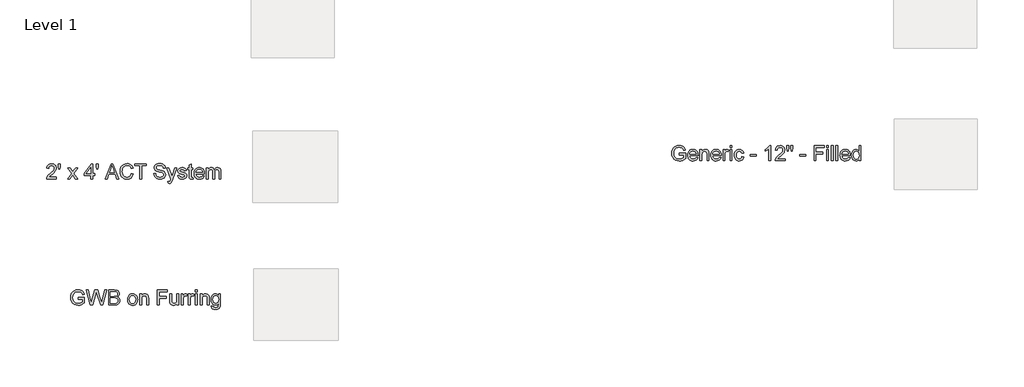
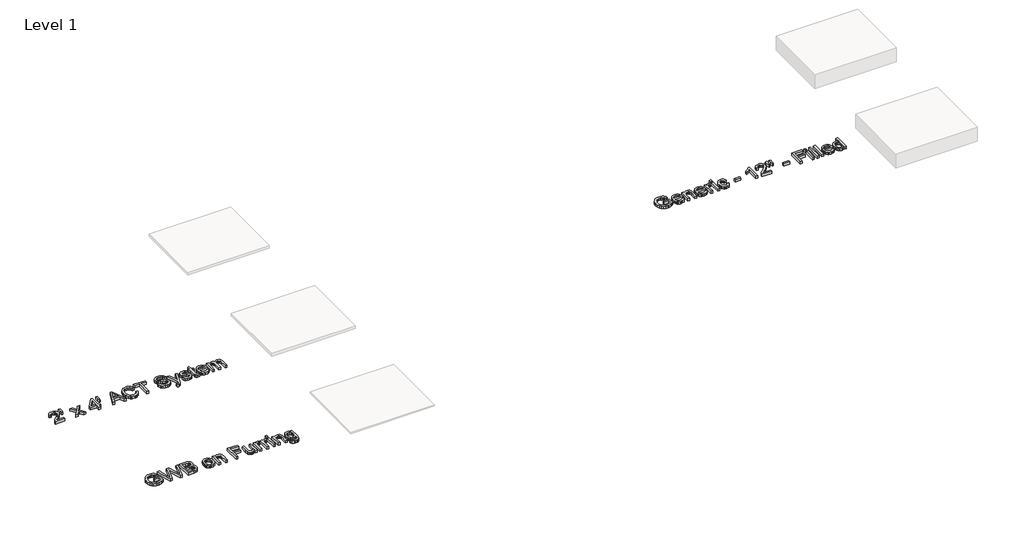
# One storey, part 10 of 42: 3 proxies.
"""IFC4 building model written with IfcOpenShell, lengths in millimetres."""

from ifc_helpers import new_model, si_unit, origin, origin_with_axes, place, context, project, spatial, polyline, outline, extrude, element, save

model = new_model("IFC4")

# Units and contexts
model_context = context("Model", 3, world=origin())
ifc_project = project(units=[si_unit("LENGTHUNIT", "METRE", prefix="MILLI")], contexts=[model_context])

# Site, building, storey
site = spatial("IfcSite", under=ifc_project)
building = spatial("IfcBuilding", under=site)
storey = spatial("IfcBuildingStorey", under=building, Name="Level 1", Elevation=0.0)

# Proxies
placement = place(None, origin())
element("IfcBuildingElementProxy", 1, Name="8\" Arial", ObjectType="8\" Arial", at=placement, inside=storey, context=model_context, shape_type="SweptSolid", body=[
    extrude(outline(polyline([(6877.2165005, -16820.3840044), (6877.2165005, -16858.4548912), (6677.3443451, -16858.4548912), (6681.4339911, -16832.2067993), (6690.8215877, -16811.6935066), (6704.5590805, -16791.7936607), (6724.4310424, -16770.9643499), (6752.2220462, -16747.6626621), (6793.3043995, -16711.1718659), (6817.9538116, -16684.2359699), (6830.2785176, -16662.3749529), (6834.3867529, -16641.1087935), (6830.5108838, -16622.0454662), (6818.8832766, -16606.1980878), (6801.0096645, -16595.5185348), (6778.3957808, -16591.9586839), (6754.6479498, -16595.434883), (6736.1980694, -16605.8634804), (6724.2916226, -16622.4265468), (6720.1740927, -16644.3061532), (6682.1032059, -16639.5472923), (6685.3772464, -16619.8937547), (6691.3327934, -16602.7218887), (6699.969847, -16588.0316942), (6711.2884072, -16575.8231713), (6725.0282237, -16566.2264451), (6740.9290463, -16559.3716407), (6779.21371, -16553.8877971), (6799.6177906, -16555.4121197), (6817.7772132, -16559.9850876), (6833.6919778, -16567.6067006), (6847.3620845, -16578.2769589), (6858.3413899, -16591.2058172), (6866.1837509, -16605.6032302), (6870.8891675, -16621.4691979), (6872.4576397, -16638.8037203), (6870.7660134, -16657.0119398), (6865.6911344, -16674.9041412), (6856.6846185, -16693.1030661), (6843.1980812, -16712.231456), (6821.6995556, -16735.0684113), (6788.6570745, -16764.3930323), (6744.8606833, -16801.0139536), (6727.6841699, -16820.3840044), (6877.2165005, -16820.3840044)])), origin_with_axes(), (0.0, 0.0, 1.0), 50.8),
    extrude(outline(polyline([(6923.8384654, -16663.3415965), (6915.2873873, -16605.5660516), (6915.2873873, -16553.8877971), (6953.3582741, -16553.8877971), (6953.3582741, -16605.5660516), (6944.43541, -16663.3415965), (6923.8384654, -16663.3415965)])), origin_with_axes(), (0.0, 0.0, 1.0), 50.8),
    extrude(outline(polyline([(7100.8829602, -16858.4548912), (7182.2297378, -16746.0268037), (7105.6418211, -16634.7884315), (7151.4458567, -16634.7884315), (7188.4013855, -16688.325616), (7205.652256, -16713.6070642), (7220.5980534, -16692.9357624), (7262.684229, -16634.7884315), (7308.4882646, -16634.7884315), (7228.0337734, -16746.0268037), (7305.5139766, -16858.4548912), (7259.7099409, -16858.4548912), (7213.0879761, -16790.8641957), (7204.536898, -16778.5209004), (7146.6869959, -16858.4548912), (7100.8829602, -16858.4548912)])), origin_with_axes(), (0.0, 0.0, 1.0), 50.8),
    extrude(outline(polyline([(7572.0101839, -16858.4548912), (7572.0101839, -16787.0719785), (7434.0032194, -16787.0719785), (7434.0032194, -16749.0010917), (7581.5279056, -16558.6466579), (7610.0810706, -16558.6466579), (7610.0810706, -16749.0010917), (7648.1519574, -16749.0010917), (7648.1519574, -16787.0719785), (7610.0810706, -16787.0719785), (7610.0810706, -16858.4548912), (7572.0101839, -16858.4548912)]), holes=[polyline([(7572.0101839, -16749.0010917), (7572.0101839, -16631.3680002), (7480.8482558, -16749.0010917), (7572.0101839, -16749.0010917)])]), origin_with_axes(), (0.0, 0.0, 1.0), 50.8),
    extrude(outline(polyline([(7690.0150614, -16663.3415965), (7681.4639833, -16605.5660516), (7681.4639833, -16553.8877971), (7719.5348701, -16553.8877971), (7719.5348701, -16605.5660516), (7710.612006, -16663.3415965), (7690.0150614, -16663.3415965)])), origin_with_axes(), (0.0, 0.0, 1.0), 50.8),
    extrude(outline(polyline([(7860.1443366, -16858.4548912), (7981.7183597, -16553.8877971), (8014.1380992, -16553.8877971), (8135.7121224, -16858.4548912), (8095.4848768, -16858.4548912), (8060.6113497, -16763.2776743), (7935.1707521, -16763.2776743), (7900.3715822, -16858.4548912), (7860.1443366, -16858.4548912)]), holes=[polyline([(7949.1499058, -16725.2067875), (8046.7065531, -16725.2067875), (8019.2687461, -16650.3290864), (7997.9282295, -16591.9586839), (7978.9671433, -16643.7856527), (7949.1499058, -16725.2067875)])]), origin_with_axes(), (0.0, 0.0, 1.0), 50.8),
    extrude(outline(polyline([(8390.5342492, -16750.190807), (8428.6051359, -16760.0059574), (8421.071822, -16783.6817549), (8411.0382473, -16804.3693223), (8398.5044116, -16822.0686597), (8383.4703151, -16836.7797672), (8366.2752125, -16848.3446355), (8347.2583584, -16856.6052558), (8326.4197529, -16861.561628), (8303.759396, -16863.213752), (8259.6005134, -16858.2132303), (8240.929885, -16851.9625781), (8224.5317986, -16843.211665), (8197.6516706, -16818.7295567), (8178.0585482, -16785.2874057), (8166.0963335, -16745.9710358), (8162.1089286, -16703.8662709), (8166.6168339, -16659.4564328), (8180.1405498, -16621.1067065), (8201.9736829, -16590.0346913), (8231.4098397, -16567.4579862), (8266.3205454, -16553.7111988), (8304.5773252, -16549.1289363), (8326.3523667, -16550.6114329), (8346.3195987, -16555.058923), (8364.4790213, -16562.4714065), (8380.8306345, -16572.8488833), (8395.1048934, -16585.9171613), (8407.0322531, -16601.4020484), (8423.8462751, -16639.6216495), (8385.7753883, -16648.693228), (8372.5769852, -16620.9301082), (8354.545364, -16601.8853702), (8331.4574532, -16590.8712098), (8303.0901812, -16587.199823), (8270.3916022, -16591.2708798), (8243.5300634, -16603.48405), (8223.1468958, -16622.5566719), (8209.8834301, -16647.206084), (8202.6057191, -16675.0714449), (8200.1798154, -16703.7919137), (8203.0518623, -16738.9628696), (8211.6680029, -16769.3749647), (8226.35355, -16793.8663677), (8247.4338164, -16811.2752473), (8272.70597, -16821.6759608), (8299.9671787, -16825.1428653), (8331.7455874, -16820.421183), (8358.2260455, -16806.2561363), (8378.2188378, -16782.7964395), (8390.5342492, -16750.190807)])), origin_with_axes(), (0.0, 0.0, 1.0), 50.8),
    extrude(outline(polyline([(8557.0943788, -16858.4548912), (8557.0943788, -16591.9586839), (8457.158301, -16591.9586839), (8457.158301, -16553.8877971), (8695.1013433, -16553.8877971), (8695.1013433, -16591.9586839), (8595.1652655, -16591.9586839), (8595.1652655, -16858.4548912), (8557.0943788, -16858.4548912)])), origin_with_axes(), (0.0, 0.0, 1.0), 50.8),
    extrude(outline(polyline([(8842.6260294, -16753.7599526), (8880.6969162, -16753.7599526), (8885.0654017, -16774.8866922), (8892.9658543, -16791.8680179), (8905.2905603, -16805.3452606), (8922.9318062, -16815.959751), (8944.4953944, -16822.8470867), (8968.5871274, -16825.1428653), (8989.7975189, -16823.4047657), (9008.3682298, -16818.190467), (9023.4162683, -16809.9368177), (9034.0586426, -16799.0806664), (9040.3882994, -16786.6165406), (9042.4981849, -16773.538968), (9040.9180944, -16760.7960027), (9036.1778229, -16749.7818423), (9026.5485654, -16740.3849511), (9010.301517, -16732.4937932), (8954.8682239, -16717.9569604), (8918.4796688, -16708.3369976), (8895.1965703, -16699.1817673), (8876.2447788, -16686.3737395), (8862.8140094, -16670.8516738), (8854.8113157, -16652.9501777), (8852.1437511, -16633.0038586), (8855.4433519, -16610.7059931), (8865.3421543, -16589.9138608), (8881.579908, -16572.2912043), (8903.8963628, -16559.5017658), (8930.6835444, -16551.7221436), (8960.3334782, -16549.1289363), (8992.4557889, -16551.8429741), (9020.5628107, -16559.9850876), (9043.6507215, -16573.387973), (9060.7156991, -16591.8843267), (9071.5160825, -16614.321612), (9075.8102108, -16639.5472923), (9037.7393241, -16639.5472923), (9030.7497472, -16616.8311675), (9016.1757359, -16600.4354047), (8993.4038432, -16590.5087184), (8961.8206222, -16587.199823), (8929.4938292, -16590.4715398), (8907.3167941, -16600.2866903), (8894.4901769, -16614.7305766), (8890.2146379, -16631.8885006), (8893.2446938, -16646.5182799), (8902.3348616, -16658.2853069), (8923.8240926, -16668.8068508), (8964.4974814, -16679.5514663), (9006.4721212, -16689.7569921), (9031.8651052, -16698.6612669), (9053.5681132, -16712.4731169), (9068.7090982, -16729.5195052), (9077.6040783, -16749.6145386), (9080.5690717, -16772.5723244), (9077.1579351, -16796.0413158), (9066.9245254, -16818.1161098), (9050.2871017, -16837.1143746), (9027.6639234, -16851.3537785), (9000.4584826, -16860.2487586), (8970.0742714, -16863.213752), (8932.7748406, -16860.0163924), (8902.0746114, -16850.4243135), (8877.620387, -16834.4003367), (8859.0589708, -16811.9072835), (8847.1432294, -16784.5066551), (8842.6260294, -16753.7599526)])), origin_with_axes(), (0.0, 0.0, 1.0), 50.8),
    extrude(outline(polyline([(9132.916541, -16944.1143864), (9128.1576801, -16907.4562864), (9147.4905523, -16910.8023605), (9165.5593521, -16906.6011786), (9176.638575, -16894.8899195), (9187.0485831, -16866.8572549), (9190.0228711, -16857.636962), (9109.1222368, -16634.7884315), (9149.2751251, -16634.7884315), (9192.1792299, -16758.9649566), (9207.1250273, -16808.6355667), (9222.0708246, -16764.7648183), (9266.1646446, -16634.7884315), (9306.0201042, -16634.7884315), (9228.1681151, -16863.8086096), (9207.9429565, -16913.4792197), (9197.5887163, -16929.3358927), (9185.8588679, -16940.3221691), (9172.2329108, -16946.7354777), (9156.1903448, -16948.8732472), (9132.916541, -16944.1143864)])), origin_with_axes(), (0.0, 0.0, 1.0), 50.8),
    extrude(outline(polyline([(9323.2709748, -16791.8308393), (9361.3418615, -16787.0719785), (9367.3462055, -16803.3562055), (9378.9645181, -16815.3277148), (9396.2711566, -16822.6890776), (9419.3404781, -16825.1428653), (9442.1309601, -16822.8935599), (9458.1549368, -16816.145644), (9467.6354799, -16806.3676721), (9470.795661, -16795.028199), (9467.6168906, -16785.3245843), (9458.0805796, -16777.9260428), (9418.8943349, -16767.0698915), (9361.5649331, -16748.4434127), (9347.0559843, -16739.0837001), (9336.5437351, -16726.6939315), (9330.1583105, -16712.0641523), (9328.0298356, -16695.9844076), (9329.7400512, -16681.233798), (9334.8706981, -16667.6171356), (9342.9570437, -16655.6735102), (9353.5343555, -16645.9420116), (9377.7376243, -16634.6768957), (9410.4919712, -16630.0295706), (9435.2715083, -16631.8977953), (9456.8165072, -16637.5024693), (9474.141735, -16646.2952083), (9486.2619587, -16657.7276279), (9494.2925364, -16672.6455413), (9499.348826, -16691.8947616), (9461.2779393, -16696.6536224), (9456.4726052, -16684.6728185), (9446.9641781, -16675.6477132), (9432.6597116, -16669.9872713), (9413.4662592, -16668.1004574), (9391.6052422, -16669.9036195), (9377.0312309, -16675.3131058), (9368.8333495, -16683.1206119), (9366.1007224, -16692.1178332), (9370.6365116, -16703.1970561), (9384.8387369, -16711.5994198), (9417.6302625, -16719.7043547), (9473.5096988, -16737.62444), (9488.2696031, -16746.1941074), (9499.4603618, -16757.9239558), (9506.5150012, -16772.8511639), (9508.8665477, -16791.0129101), (9506.1060366, -16809.7881033), (9497.8245034, -16827.4479385), (9484.3379661, -16842.6075128), (9465.9624429, -16853.8819233), (9443.7668185, -16860.8807948), (9418.8199777, -16863.213752), (9380.4330728, -16858.7151414), (9352.4189974, -16845.2193094), (9333.7181615, -16822.8749706), (9323.2709748, -16791.8308393)])), origin_with_axes(), (0.0, 0.0, 1.0), 50.8),
    extrude(outline(polyline([(9632.5969297, -16826.7043665), (9637.3557905, -16859.5702492), (9608.8769827, -16863.213752), (9590.6037006, -16861.6336615), (9576.9777436, -16856.89339), (9567.3484861, -16849.587795), (9561.0653026, -16840.3117342), (9557.6076928, -16824.380704), (9556.4551562, -16797.1102006), (9556.4551562, -16672.8593182), (9527.9019911, -16672.8593182), (9527.9019911, -16634.7884315), (9556.4551562, -16634.7884315), (9556.4551562, -16580.4333178), (9594.5260429, -16558.0518003), (9594.5260429, -16634.7884315), (9632.5969297, -16634.7884315), (9632.5969297, -16672.8593182), (9594.5260429, -16672.8593182), (9594.5260429, -16795.9948426), (9596.5336873, -16815.6251436), (9603.0399424, -16822.5775418), (9616.0152739, -16825.1428653), (9632.5969297, -16826.7043665)])), origin_with_axes(), (0.0, 0.0, 1.0), 50.8),
    extrude(outline(polyline([(9827.2640811, -16791.8308393), (9864.5913959, -16796.5897002), (9851.1420372, -16824.7153114), (9829.6806901, -16845.7398099), (9800.6906765, -16858.8452665), (9764.6553181, -16863.213752), (9741.0329649, -16861.3292617), (9719.9852298, -16855.6757908), (9701.5121128, -16846.2533393), (9685.6136138, -16833.0619071), (9672.8288226, -16816.4686331), (9663.6968289, -16796.8406557), (9658.2176326, -16774.1779752), (9656.3912339, -16748.4805913), (9658.2362219, -16721.9118341), (9663.7711861, -16698.4939632), (9672.9961263, -16678.2269786), (9685.9110426, -16661.1108805), (9701.7677156, -16647.5128074), (9719.8179261, -16637.7998981), (9740.061674, -16631.9721525), (9762.4989593, -16630.0295706), (9784.2135856, -16631.9675052), (9803.8508575, -16637.7813088), (9821.4107752, -16647.4709815), (9836.8933386, -16661.0365233), (9849.5317391, -16678.1154428), (9858.559168, -16698.3452488), (9863.9756253, -16721.7259411), (9865.7811111, -16748.2575197), (9865.5580395, -16758.5188134), (9694.4621207, -16758.5188134), (9701.0520276, -16787.0162106), (9716.3603163, -16807.9663519), (9738.4536995, -16820.8487369), (9765.3988901, -16825.1428653), (9785.6612273, -16823.1538101), (9802.7262049, -16817.1866448), (9816.5938228, -16806.8695832), (9827.2640811, -16791.8308393)]), holes=[polyline([(9694.4621207, -16720.4479267), (9827.7102243, -16720.4479267), (9822.5609882, -16700.3343039), (9812.4669982, -16685.9461855), (9790.2713738, -16672.5618894), (9762.3502449, -16668.1004574), (9736.687716, -16671.6603084), (9715.4680299, -16682.3398613), (9700.7174202, -16698.9865796), (9694.4621207, -16720.4479267)])]), origin_with_axes(), (0.0, 0.0, 1.0), 50.8),
    extrude(outline(polyline([(9903.8519978, -16858.4548912), (9903.8519978, -16634.7884315), (9941.9228846, -16634.7884315), (9941.9228846, -16671.5952458), (9953.3738935, -16654.6882773), (9968.0966192, -16641.4434009), (9985.5891507, -16632.8830282), (10005.3495768, -16630.0295706), (10026.5227897, -16632.9387961), (10043.4948208, -16641.6664725), (10056.1727235, -16655.6363316), (10064.4635513, -16674.272105), (10078.3404639, -16654.9159962), (10094.169253, -16641.0902042), (10111.9499186, -16632.794729), (10131.6824608, -16630.0295706), (10160.3006884, -16634.6304224), (10181.4646067, -16648.4329778), (10194.5421793, -16671.8090228), (10198.9013702, -16705.1303433), (10198.9013702, -16858.4548912), (10160.8304835, -16858.4548912), (10160.8304835, -16721.4889275), (10157.2985164, -16689.7012242), (10152.3351733, -16680.9363691), (10144.5090779, -16674.0490334), (10134.4429719, -16669.5876014), (10122.7595967, -16668.1004574), (10102.1347682, -16671.9112639), (10085.3207461, -16683.3436835), (10074.1392821, -16703.1784668), (10070.4121274, -16732.1963644), (10070.4121274, -16858.4548912), (10032.3412406, -16858.4548912), (10032.3412406, -16717.250567), (10030.1384086, -16695.7241574), (10023.5299124, -16680.3693955), (10011.9023051, -16671.1676919), (9994.6421399, -16668.1004574), (9979.9751821, -16670.1452804), (9966.4607608, -16676.2797495), (9955.3071807, -16686.3551502), (9947.7227463, -16700.2227681), (9943.37285, -16719.4626938), (9941.9228846, -16745.6550177), (9941.9228846, -16858.4548912), (9903.8519978, -16858.4548912)])), origin_with_axes(), (0.0, 0.0, 1.0), 50.8),
])
element("IfcBuildingElementProxy", 2, Name="8\" Arial", ObjectType="8\" Arial", at=placement, inside=storey, context=model_context, shape_type="SweptSolid", body=[
    extrude(outline(polyline([(7319.6329177, -19290.0141217), (7319.6329177, -19251.943235), (7443.3632997, -19251.943235), (7443.3632997, -19365.7841092), (7413.2951067, -19386.6970719), (7382.2788593, -19401.6986372), (7350.3889149, -19410.7330371), (7317.6996305, -19413.7445037), (7274.9907134, -19408.9577589), (7236.3900315, -19394.5975245), (7204.3234887, -19371.1657116), (7181.2169886, -19339.1642314), (7167.2471295, -19300.7773265), (7162.5905098, -19258.1892398), (7167.2285402, -19215.2944297), (7181.1426314, -19175.3924968), (7203.7565151, -19141.9224619), (7218.1097785, -19128.8890388), (7234.4939229, -19118.3233453), (7271.9327735, -19104.3256023), (7314.6509853, -19099.6596879), (7346.0111347, -19102.3644311), (7374.211103, -19110.4786606), (7397.958934, -19123.4168135), (7415.9626712, -19140.5933269), (7429.2819048, -19162.8354246), (7438.9762248, -19190.9703304), (7403.8796261, -19200.8598381), (7396.0442361, -19180.7926885), (7386.5172198, -19165.6517035), (7373.9136742, -19154.2378732), (7356.8486967, -19145.3521878), (7336.5027076, -19139.635978), (7314.0561277, -19137.7305747), (7287.7801519, -19139.7846924), (7265.3149826, -19145.9470454), (7246.7442717, -19155.4461778), (7232.1516711, -19167.5106336), (7212.5585487, -19196.8445492), (7203.6356846, -19225.5836073), (7200.6613966, -19256.6277386), (7204.2398369, -19293.034883), (7214.9751577, -19322.9915402), (7232.5420464, -19346.2839333), (7256.6151901, -19362.6982854), (7284.7872745, -19372.429784), (7314.6509853, -19375.6736169), (7341.0199076, -19373.229124), (7366.7382044, -19365.895645), (7389.0732485, -19355.7923604), (7405.2924129, -19345.0384502), (7405.2924129, -19290.0141217), (7319.6329177, -19290.0141217)])), origin_with_axes(), (0.0, 0.0, 1.0), 50.8),
    extrude(outline(polyline([(7559.7323188, -19408.9856428), (7476.6753256, -19104.4185488), (7515.9359276, -19104.4185488), (7564.1193936, -19304.5881331), (7578.9908338, -19366.3789668), (7594.9032747, -19311.7264243), (7655.2813217, -19104.4185488), (7711.8671514, -19104.4185488), (7755.7378998, -19254.6944514), (7774.5316823, -19310.4623519), (7788.3807109, -19366.3789668), (7802.8060079, -19306.3727059), (7851.4356171, -19104.4185488), (7890.6962191, -19104.4185488), (7807.5648687, -19408.9856428), (7766.8914799, -19408.9856428), (7693.8727088, -19174.0168886), (7683.6857724, -19141.2253631), (7672.2347634, -19180.7090367), (7605.6850688, -19408.9856428), (7559.7323188, -19408.9856428)])), origin_with_axes(), (0.0, 0.0, 1.0), 50.8),
    extrude(outline(polyline([(7928.7671059, -19408.9856428), (7928.7671059, -19104.4185488), (8044.9874106, -19104.4185488), (8076.9517122, -19106.6585594), (8101.9078477, -19113.3785915), (8121.0362376, -19124.7459485), (8135.5173024, -19140.9279343), (8144.6353541, -19159.9633777), (8147.6747047, -19179.8911075), (8145.1186759, -19198.2294521), (8137.4505896, -19215.471028), (8124.6146779, -19230.5562451), (8106.5551727, -19242.4255133), (8128.1280556, -19253.6906292), (8144.0683805, -19270.8299639), (8153.9114149, -19292.7095702), (8157.1924264, -19318.1955008), (8154.9524157, -19339.4337762), (8148.2323837, -19359.1291398), (8138.2034563, -19375.8780992), (8126.0367593, -19388.2771624), (8111.1374352, -19397.2557944), (8092.9106264, -19403.7434602), (8044.0951241, -19408.9856428), (7928.7671059, -19408.9856428)]), holes=[polyline([(7966.8379926, -19228.1489307), (8036.3619753, -19228.1489307), (8076.9610069, -19224.8772139), (8091.1725268, -19219.2353613), (8101.3873473, -19210.7865244), (8107.5497003, -19199.6608282), (8109.603818, -19185.9883979), (8107.68912, -19172.7156376), (8101.9450263, -19161.1530929), (8092.6317869, -19152.1279877), (8080.0096521, -19146.4675458), (8031.082614, -19142.4894355), (7966.8379926, -19142.4894355), (7966.8379926, -19228.1489307)]), polyline([(7966.8379926, -19370.9147561), (8044.9130534, -19370.9147561), (8073.1687896, -19369.4276121), (8097.0746296, -19361.1367842), (8112.9127134, -19344.220521), (8117.5693331, -19332.267601), (8119.1215397, -19318.5672868), (8117.2997882, -19302.6548458), (8111.834534, -19288.9731209), (8102.2889283, -19278.2749787), (8088.2261228, -19271.3132857), (8068.3076876, -19267.4931846), (8041.1951933, -19266.2198175), (7966.8379926, -19266.2198175), (7966.8379926, -19370.9147561)])]), origin_with_axes(), (0.0, 0.0, 1.0), 50.8),
    extrude(outline(polyline([(8314.2348343, -19297.152413), (8316.2935993, -19268.185636), (8322.4698943, -19243.2248532), (8332.7637192, -19222.2700646), (8347.1750742, -19205.3212701), (8361.684023, -19194.4883554), (8377.6987051, -19186.7505592), (8395.2191205, -19182.1078815), (8414.2452692, -19180.5603223), (8435.2488548, -19182.4448126), (8454.2401486, -19188.0982835), (8471.2191506, -19197.520735), (8486.1858609, -19210.7121672), (8498.4013548, -19227.2264367), (8507.1267076, -19246.6174005), (8512.3619192, -19268.8850584), (8514.1069898, -19294.0294106), (8511.0211659, -19332.4906726), (8501.7636945, -19361.7688204), (8486.6041202, -19383.6948999), (8465.8119879, -19400.0999574), (8441.1161026, -19410.3333671), (8414.2452692, -19413.7445037), (8392.9349602, -19411.8669844), (8373.7670681, -19406.2344264), (8356.7415928, -19396.8468298), (8341.8585343, -19383.7041946), (8329.7731656, -19367.0295923), (8321.1407593, -19347.0460947), (8315.9613155, -19323.7537015), (8314.2348343, -19297.152413)]), holes=[polyline([(8352.305721, -19297.0780558), (8356.7113852, -19331.5333237), (8369.9283776, -19356.0804945), (8389.8189288, -19370.7753363), (8414.2452692, -19375.6736169), (8438.5600739, -19370.7474524), (8458.4134464, -19355.9689587), (8471.6304389, -19331.0964751), (8476.036103, -19295.8883406), (8471.6025549, -19262.4368949), (8458.3019106, -19238.2243314), (8438.4206541, -19223.5294896), (8414.2452692, -19218.631209), (8389.8189288, -19223.5109003), (8369.9283776, -19238.1499742), (8356.7113852, -19262.6413772), (8352.305721, -19297.0780558)])]), origin_with_axes(), (0.0, 0.0, 1.0), 50.8),
    extrude(outline(polyline([(8556.9367374, -19408.9856428), (8556.9367374, -19185.3191831), (8595.0076241, -19185.3191831), (8595.0076241, -19216.5492074), (8608.2339112, -19200.8040702), (8624.1184682, -19189.5575436), (8642.6612951, -19182.8096276), (8663.862392, -19180.5603223), (8682.6282905, -19182.3727791), (8699.8140985, -19187.8101494), (8714.146449, -19196.1939237), (8724.3519748, -19206.8455927), (8735.7658051, -19234.8410788), (8737.7734495, -19271.6478931), (8737.7734495, -19408.9856428), (8699.7025627, -19408.9856428), (8699.7025627, -19276.77854), (8695.3154879, -19243.0947281), (8689.2460814, -19233.0658006), (8679.8120115, -19225.2861785), (8667.7196718, -19220.2949514), (8653.6754555, -19218.631209), (8631.3775899, -19222.3676584), (8612.3700305, -19233.5770064), (8604.7739777, -19242.7275894), (8599.3482257, -19255.2335411), (8595.0076241, -19290.3115505), (8595.0076241, -19408.9856428), (8556.9367374, -19408.9856428)])), origin_with_axes(), (0.0, 0.0, 1.0), 50.8),
    extrude(outline(polyline([(8913.8513007, -19408.9856428), (8913.8513007, -19104.4185488), (9118.4823171, -19104.4185488), (9118.4823171, -19142.4894355), (8951.9221875, -19142.4894355), (8951.9221875, -19232.9077916), (9094.6880128, -19232.9077916), (9094.6880128, -19270.9786783), (8951.9221875, -19270.9786783), (8951.9221875, -19408.9856428), (8913.8513007, -19408.9856428)])), origin_with_axes(), (0.0, 0.0, 1.0), 50.8),
    extrude(outline(polyline([(9308.8367509, -19408.9856428), (9308.8367509, -19370.5429701), (9295.0620794, -19389.443641), (9279.0195134, -19402.9441203), (9260.7090527, -19411.0444078), (9240.1306974, -19413.7445037), (9221.5878705, -19411.8483951), (9204.3277053, -19406.1600692), (9189.8466404, -19397.6089911), (9179.6411146, -19387.1246258), (9172.7723682, -19374.3909552), (9168.3016415, -19359.0919612), (9166.0709255, -19323.6979336), (9166.0709255, -19185.3191831), (9204.1418123, -19185.3191831), (9204.1418123, -19305.7778483), (9206.4468855, -19344.592307), (9211.9957916, -19357.5397546), (9221.5042186, -19367.382789), (9234.3401304, -19373.60091), (9249.8714907, -19375.6736169), (9266.2951374, -19373.5544367), (9281.659194, -19367.196896), (9294.3278021, -19357.1865579), (9302.6651032, -19344.1089852), (9307.2938389, -19326.1981945), (9308.8367509, -19301.6882022), (9308.8367509, -19185.3191831), (9346.9076376, -19185.3191831), (9346.9076376, -19408.9856428), (9308.8367509, -19408.9856428)])), origin_with_axes(), (0.0, 0.0, 1.0), 50.8),
    extrude(outline(polyline([(9399.2551069, -19408.9856428), (9399.2551069, -19185.3191831), (9432.5671328, -19185.3191831), (9432.5671328, -19218.4081374), (9444.8732495, -19199.2239797), (9456.2127226, -19187.9216852), (9467.5893744, -19182.400663), (9480.0070269, -19180.5603223), (9498.968113, -19183.4974317), (9518.226628, -19192.30876), (9505.5115467, -19226.4387151), (9492.1272506, -19220.5830856), (9478.7429545, -19218.631209), (9467.3755974, -19220.5087284), (9457.2165449, -19226.1412863), (9449.0093688, -19235.101329), (9443.4976413, -19246.9613025), (9438.8689056, -19268.2274619), (9437.3259937, -19291.4269085), (9437.3259937, -19408.9856428), (9399.2551069, -19408.9856428)])), origin_with_axes(), (0.0, 0.0, 1.0), 50.8),
    extrude(outline(polyline([(9542.0209323, -19408.9856428), (9542.0209323, -19185.3191831), (9575.3329582, -19185.3191831), (9575.3329582, -19218.4081374), (9587.6390749, -19199.2239797), (9598.978548, -19187.9216852), (9610.3551997, -19182.400663), (9622.7728522, -19180.5603223), (9641.7339384, -19183.4974317), (9660.9924534, -19192.30876), (9648.2773721, -19226.4387151), (9634.8930759, -19220.5830856), (9621.5087798, -19218.631209), (9610.1414227, -19220.5087284), (9599.9823702, -19226.1412863), (9591.7751942, -19235.101329), (9586.2634667, -19246.9613025), (9581.6347309, -19268.2274619), (9580.091819, -19291.4269085), (9580.091819, -19408.9856428), (9542.0209323, -19408.9856428)])), origin_with_axes(), (0.0, 0.0, 1.0), 50.8),
    extrude(outline(polyline([(9684.7867576, -19142.4894355), (9684.7867576, -19104.4185488), (9722.8576444, -19104.4185488), (9722.8576444, -19142.4894355), (9684.7867576, -19142.4894355)])), origin_with_axes(), (0.0, 0.0, 1.0), 50.8),
    extrude(outline(polyline([(9684.7867576, -19408.9856428), (9684.7867576, -19185.3191831), (9722.8576444, -19185.3191831), (9722.8576444, -19408.9856428), (9684.7867576, -19408.9856428)])), origin_with_axes(), (0.0, 0.0, 1.0), 50.8),
    extrude(outline(polyline([(9779.9639745, -19408.9856428), (9779.9639745, -19185.3191831), (9818.0348613, -19185.3191831), (9818.0348613, -19216.5492074), (9831.2611483, -19200.8040702), (9847.1457053, -19189.5575436), (9865.6885323, -19182.8096276), (9886.8896291, -19180.5603223), (9905.6555276, -19182.3727791), (9922.8413356, -19187.8101494), (9937.1736861, -19196.1939237), (9947.3792119, -19206.8455927), (9958.7930422, -19234.8410788), (9960.8006866, -19271.6478931), (9960.8006866, -19408.9856428), (9922.7297998, -19408.9856428), (9922.7297998, -19276.77854), (9918.342725, -19243.0947281), (9912.2733185, -19233.0658006), (9902.8392487, -19225.2861785), (9890.7469089, -19220.2949514), (9876.7026926, -19218.631209), (9854.404827, -19222.3676584), (9835.3972676, -19233.5770064), (9827.8012148, -19242.7275894), (9822.3754628, -19255.2335411), (9818.0348613, -19290.3115505), (9818.0348613, -19408.9856428), (9779.9639745, -19408.9856428)])), origin_with_axes(), (0.0, 0.0, 1.0), 50.8),
    extrude(outline(polyline([(10003.6304342, -19428.0210862), (10041.701321, -19432.7799471), (10045.9025028, -19444.6770992), (10054.0446163, -19452.8563913), (10070.0500037, -19459.2139319), (10091.000145, -19461.3331121), (10113.3444838, -19458.9350924), (10129.9633182, -19451.7410332), (10141.4886843, -19440.2156671), (10148.5526184, -19424.8237266), (10151.1551204, -19380.4324778), (10138.4865123, -19392.9244875), (10124.3493495, -19401.8473516), (10108.743632, -19407.20107), (10091.6693598, -19408.9856428), (10070.7958994, -19406.9082885), (10052.4180525, -19400.6762257), (10036.5358192, -19390.2894542), (10023.1491994, -19375.7479741), (10012.527738, -19358.3019159), (10004.9409799, -19339.20141), (10000.388925, -19318.4464563), (9998.8715734, -19296.037055), (10001.5949058, -19265.2996471), (10009.7649033, -19237.0346162), (10023.0934315, -19213.0823029), (10041.2923564, -19195.283048), (10063.7389363, -19184.2410037), (10089.8104298, -19180.5603223), (10107.6143321, -19182.6423239), (10123.7730812, -19188.8883288), (10138.2866773, -19199.2983369), (10151.1551204, -19213.8723482), (10151.1551204, -19185.3191831), (10189.2260071, -19185.3191831), (10189.2260071, -19378.4248333), (10186.6235051, -19423.0112698), (10178.815999, -19452.3730694), (10165.3666404, -19471.8453614), (10145.8385805, -19486.7632748), (10120.6593735, -19496.2438179), (10090.256573, -19499.4039989), (10054.8346615, -19494.9518615), (10026.9414166, -19481.5954493), (10016.4361384, -19471.5688455), (10009.0492152, -19459.2975838), (10004.7806471, -19444.781664), (10003.6304342, -19428.0210862)]), holes=[polyline([(10036.9424601, -19293.4345529), (10041.0042222, -19328.3545533), (10053.1895085, -19352.3626345), (10071.5092638, -19366.2767257), (10093.9744331, -19370.9147561), (10116.2722986, -19366.3046096), (10134.6850004, -19352.4741703), (10147.0375904, -19328.7728126), (10151.1551204, -19294.549911), (10146.9167599, -19261.5446085), (10134.2016786, -19237.7781882), (10115.519432, -19223.4179538), (10093.3795754, -19218.631209), (10071.6393889, -19223.3435966), (10053.4125801, -19237.4807594), (10041.0599901, -19260.893983), (10036.9424601, -19293.4345529)])]), origin_with_axes(), (0.0, 0.0, 1.0), 50.8),
])
element("IfcBuildingElementProxy", 3, Name="8\" Arial", ObjectType="8\" Arial", at=placement, inside=storey, context=model_context, shape_type="SweptSolid", body=[
    extrude(outline(polyline([(19456.3608606, -16371.1352359), (19456.3608606, -16333.0643492), (19580.0912426, -16333.0643492), (19580.0912426, -16446.9052234), (19550.0230495, -16467.8181861), (19519.0068022, -16482.8197514), (19487.1168577, -16491.8541513), (19454.4275734, -16494.8656179), (19411.7186562, -16490.0788731), (19373.1179744, -16475.7186387), (19341.0514316, -16452.2868258), (19317.9449315, -16420.2853456), (19303.9750724, -16381.8984407), (19299.3184527, -16339.310354), (19303.9564831, -16296.4155439), (19317.8705743, -16256.5136111), (19340.484458, -16223.0435761), (19354.8377214, -16210.010153), (19371.2218658, -16199.4444595), (19408.6607164, -16185.4467165), (19451.3789282, -16180.7808021), (19482.7390776, -16183.4855453), (19510.9390459, -16191.5997748), (19534.6868769, -16204.5379278), (19552.6906141, -16221.7144411), (19566.0098477, -16243.9565388), (19575.7041677, -16272.0914446), (19540.607569, -16281.9809523), (19532.772179, -16261.9138028), (19523.2451626, -16246.7728178), (19510.6416171, -16235.3589875), (19493.5766396, -16226.473302), (19473.2306505, -16220.7570922), (19450.7840706, -16218.8516889), (19424.5080948, -16220.9058066), (19402.0429255, -16227.0681596), (19383.4722146, -16236.567292), (19368.879614, -16248.6317478), (19349.2864916, -16277.9656635), (19340.3636275, -16306.7047215), (19337.3893395, -16337.7488528), (19340.9677798, -16374.1559972), (19351.7031006, -16404.1126544), (19369.2699893, -16427.4050476), (19393.343133, -16443.8193996), (19421.5152174, -16453.5508983), (19451.3789282, -16456.7947311), (19477.7478505, -16454.3502382), (19503.4661473, -16447.0167592), (19525.8011914, -16436.9134746), (19542.0203558, -16426.1595645), (19542.0203558, -16371.1352359), (19456.3608606, -16371.1352359)])), origin_with_axes(), (0.0, 0.0, 1.0), 50.8),
    extrude(outline(polyline([(19793.7938374, -16423.4827052), (19831.1211521, -16428.2415661), (19817.6717935, -16456.3671772), (19796.2104464, -16477.3916757), (19767.2204328, -16490.4971324), (19731.1850744, -16494.8656179), (19707.5627212, -16492.9811276), (19686.5149861, -16487.3276567), (19668.041869, -16477.9052052), (19652.1433701, -16464.713773), (19639.3585789, -16448.1204989), (19630.2265851, -16428.4925216), (19624.7473889, -16405.829841), (19622.9209902, -16380.1324572), (19624.7659782, -16353.5636999), (19630.3009423, -16330.145829), (19639.5258826, -16309.8788445), (19652.4407989, -16292.7627464), (19668.2974719, -16279.1646733), (19686.3476824, -16269.451764), (19706.5914303, -16263.6240184), (19729.0287156, -16261.6814365), (19750.7433418, -16263.619371), (19770.3806138, -16269.4331747), (19787.9405315, -16279.1228474), (19803.4230949, -16292.6883892), (19816.0614953, -16309.7673087), (19825.0889242, -16329.9971146), (19830.5053816, -16353.3778069), (19832.3108673, -16379.9093856), (19832.0877957, -16390.1706793), (19660.9918769, -16390.1706793), (19667.5817838, -16418.6680765), (19682.8900725, -16439.6182178), (19704.9834558, -16452.5006028), (19731.9286464, -16456.7947311), (19752.1909836, -16454.805676), (19769.2559612, -16448.8385107), (19783.1235791, -16438.5214491), (19793.7938374, -16423.4827052)]), holes=[polyline([(19660.9918769, -16352.0997926), (19794.2399806, -16352.0997926), (19789.0907444, -16331.9861698), (19778.9967544, -16317.5980514), (19756.80113, -16304.2137553), (19728.8800012, -16299.7523233), (19703.2174723, -16303.3121742), (19681.9977861, -16313.9917272), (19667.2471764, -16330.6384455), (19660.9918769, -16352.0997926)])]), origin_with_axes(), (0.0, 0.0, 1.0), 50.8),
    extrude(outline(polyline([(19870.3817541, -16490.1067571), (19870.3817541, -16266.4402973), (19908.4526409, -16266.4402973), (19908.4526409, -16297.6703216), (19921.6789279, -16281.9251844), (19937.5634849, -16270.6786578), (19956.1063119, -16263.9307418), (19977.3074087, -16261.6814365), (19996.0733072, -16263.4938933), (20013.2591153, -16268.9312636), (20027.5914657, -16277.315038), (20037.7969915, -16287.966707), (20049.2108218, -16315.962193), (20051.2184662, -16352.7690074), (20051.2184662, -16490.1067571), (20013.1475795, -16490.1067571), (20013.1475795, -16357.8996542), (20008.7605046, -16324.2158423), (20002.6910981, -16314.1869148), (19993.2570283, -16306.4072927), (19981.1646885, -16301.4160656), (19967.1204722, -16299.7523233), (19944.8226067, -16303.4887726), (19925.8150472, -16314.6981206), (19918.2189944, -16323.8487036), (19912.7932425, -16336.3546553), (19908.4526409, -16371.4326647), (19908.4526409, -16490.1067571), (19870.3817541, -16490.1067571)])), origin_with_axes(), (0.0, 0.0, 1.0), 50.8),
    extrude(outline(polyline([(20260.1622002, -16423.4827052), (20297.4895149, -16428.2415661), (20284.0401563, -16456.3671772), (20262.5788092, -16477.3916757), (20233.5887956, -16490.4971324), (20197.5534372, -16494.8656179), (20173.931084, -16492.9811276), (20152.8833489, -16487.3276567), (20134.4102318, -16477.9052052), (20118.5117328, -16464.713773), (20105.7269416, -16448.1204989), (20096.5949479, -16428.4925216), (20091.1157517, -16405.829841), (20089.289353, -16380.1324572), (20091.134341, -16353.5636999), (20096.6693051, -16330.145829), (20105.8942454, -16309.8788445), (20118.8091616, -16292.7627464), (20134.6658347, -16279.1646733), (20152.7160452, -16269.451764), (20172.9597931, -16263.6240184), (20195.3970784, -16261.6814365), (20217.1117046, -16263.619371), (20236.7489766, -16269.4331747), (20254.3088943, -16279.1228474), (20269.7914577, -16292.6883892), (20282.4298581, -16309.7673087), (20291.457287, -16329.9971146), (20296.8737444, -16353.3778069), (20298.6792301, -16379.9093856), (20298.4561585, -16390.1706793), (20127.3602397, -16390.1706793), (20133.9501466, -16418.6680765), (20149.2584353, -16439.6182178), (20171.3518186, -16452.5006028), (20198.2970092, -16456.7947311), (20218.5593464, -16454.805676), (20235.6243239, -16448.8385107), (20249.4919419, -16438.5214491), (20260.1622002, -16423.4827052)]), holes=[polyline([(20127.3602397, -16352.0997926), (20260.6083434, -16352.0997926), (20255.4591072, -16331.9861698), (20245.3651172, -16317.5980514), (20223.1694928, -16304.2137553), (20195.248364, -16299.7523233), (20169.5858351, -16303.3121742), (20148.3661489, -16313.9917272), (20133.6155392, -16330.6384455), (20127.3602397, -16352.0997926)])]), origin_with_axes(), (0.0, 0.0, 1.0), 50.8),
    extrude(outline(polyline([(20336.7501169, -16490.1067571), (20336.7501169, -16266.4402973), (20370.0621428, -16266.4402973), (20370.0621428, -16299.5292517), (20382.3682595, -16280.3450939), (20393.7077326, -16269.0427994), (20405.0843843, -16263.5217772), (20417.5020369, -16261.6814365), (20436.463123, -16264.6185459), (20455.721638, -16273.4298742), (20443.0065567, -16307.5598293), (20429.6222606, -16301.7041998), (20416.2379644, -16299.7523233), (20404.8706074, -16301.6298426), (20394.7115548, -16307.2624005), (20386.5043788, -16316.2224432), (20380.9926513, -16328.0824167), (20376.3639156, -16349.3485761), (20374.8210037, -16372.5480227), (20374.8210037, -16490.1067571), (20336.7501169, -16490.1067571)])), origin_with_axes(), (0.0, 0.0, 1.0), 50.8),
    extrude(outline(polyline([(20479.5159422, -16490.1067571), (20479.5159422, -16266.4402973), (20517.586829, -16266.4402973), (20517.586829, -16490.1067571), (20479.5159422, -16490.1067571)])), origin_with_axes(), (0.0, 0.0, 1.0), 50.8),
    extrude(outline(polyline([(20479.5159422, -16223.6105497), (20479.5159422, -16185.539663), (20517.586829, -16185.539663), (20517.586829, -16223.6105497), (20479.5159422, -16223.6105497)])), origin_with_axes(), (0.0, 0.0, 1.0), 50.8),
    extrude(outline(polyline([(20717.4589845, -16409.2061227), (20755.5298712, -16413.9649835), (20744.9153808, -16447.8253938), (20724.9690618, -16473.4135655), (20697.5684333, -16489.5026048), (20664.5910148, -16494.8656179), (20643.2388799, -16492.9950696), (20624.0942244, -16487.3834246), (20607.1570482, -16478.0306829), (20592.4273515, -16464.9368446), (20580.5046391, -16448.3482179), (20571.988416, -16428.5111109), (20566.8786821, -16405.4255238), (20565.1754375, -16379.0914564), (20568.0846629, -16345.2124568), (20576.8123394, -16315.8506572), (20591.4978865, -16292.1400048), (20612.2807241, -16275.214447), (20637.1439131, -16265.0646891), (20664.0705144, -16261.6814365), (20696.2392983, -16266.3287615), (20721.9575951, -16280.2707367), (20740.4074756, -16302.7637899), (20750.7710104, -16333.0643492), (20712.7001236, -16337.82321), (20705.7941986, -16321.2136703), (20695.0402885, -16309.3072236), (20681.0332508, -16302.1410483), (20664.3679432, -16299.7523233), (20639.7650044, -16304.4554162), (20620.2369446, -16318.564695), (20607.4939793, -16342.8423211), (20603.2463242, -16378.0504556), (20607.4010328, -16413.7326173), (20619.8651586, -16438.0938952), (20639.0400217, -16452.1195221), (20663.3269424, -16456.7947311), (20683.0408952, -16453.876211), (20699.2042917, -16445.1206506), (20710.9620241, -16430.3049784), (20717.4589845, -16409.2061227)])), origin_with_axes(), (0.0, 0.0, 1.0), 50.8),
    extrude(outline(polyline([(20888.7779749, -16399.688401), (20888.7779749, -16361.6175142), (21007.749496, -16361.6175142), (21007.749496, -16399.688401), (20888.7779749, -16399.688401)])), origin_with_axes(), (0.0, 0.0, 1.0), 50.8),
    extrude(outline(polyline([(21302.7988684, -16490.1067571), (21264.7279816, -16490.1067571), (21264.7279816, -16252.7585724), (21228.6647393, -16278.4489853), (21188.5862081, -16297.6703216), (21188.5862081, -16261.6814365), (21218.4870975, -16245.4157989), (21244.3912872, -16226.0643374), (21264.8116335, -16205.4859821), (21278.2609922, -16185.539663), (21302.7988684, -16185.539663), (21302.7988684, -16490.1067571)])), origin_with_axes(), (0.0, 0.0, 1.0), 50.8),
    extrude(outline(polyline([(21588.3305191, -16452.0358703), (21588.3305191, -16490.1067571), (21388.4583636, -16490.1067571), (21392.5480096, -16463.8586652), (21401.9356062, -16443.3453725), (21415.6730991, -16423.4455266), (21435.5450609, -16402.6162158), (21463.3360647, -16379.314528), (21504.4184181, -16342.8237318), (21529.0678301, -16315.8878358), (21541.3925361, -16294.0268188), (21545.5007715, -16272.7606594), (21541.6249024, -16253.6973321), (21529.9972951, -16237.8499537), (21512.123683, -16227.1704007), (21489.5097994, -16223.6105497), (21465.7619684, -16227.0867489), (21447.312088, -16237.5153463), (21435.4056412, -16254.0784127), (21431.2881112, -16275.958019), (21393.2172244, -16271.1991582), (21396.4912649, -16251.5456206), (21402.446812, -16234.3737545), (21411.0838656, -16219.6835601), (21422.4024257, -16207.4750372), (21436.1422422, -16197.878311), (21452.0430649, -16191.0235065), (21490.3277286, -16185.539663), (21510.7318092, -16187.0639856), (21528.8912318, -16191.6369534), (21544.8059964, -16199.2585665), (21558.476103, -16209.9288248), (21569.4554084, -16222.8576831), (21577.2977694, -16237.2550961), (21582.003186, -16253.1210638), (21583.5716582, -16270.4555862), (21581.8800319, -16288.6638057), (21576.805153, -16306.5560071), (21567.798637, -16324.754932), (21554.3120998, -16343.8833219), (21532.8135741, -16366.7202771), (21499.7710931, -16396.0448982), (21455.9747018, -16432.6658195), (21438.7981885, -16452.0358703), (21588.3305191, -16452.0358703)])), origin_with_axes(), (0.0, 0.0, 1.0), 50.8),
    extrude(outline(polyline([(21635.6960559, -16294.9934624), (21626.4014058, -16236.1769167), (21626.4014058, -16185.539663), (21664.4722926, -16185.539663), (21664.4722926, -16236.1769167), (21656.1442861, -16294.9934624), (21635.6960559, -16294.9934624)])), origin_with_axes(), (0.0, 0.0, 1.0), 50.8),
    extrude(outline(polyline([(21711.6147578, -16294.9934624), (21702.5431794, -16236.1769167), (21702.5431794, -16185.539663), (21740.6140661, -16185.539663), (21740.6140661, -16236.1769167), (21731.691202, -16294.9934624), (21711.6147578, -16294.9934624)])), origin_with_axes(), (0.0, 0.0, 1.0), 50.8),
    extrude(outline(polyline([(21888.1387523, -16399.688401), (21888.1387523, -16361.6175142), (22007.1102734, -16361.6175142), (22007.1102734, -16399.688401), (21888.1387523, -16399.688401)])), origin_with_axes(), (0.0, 0.0, 1.0), 50.8),
    extrude(outline(polyline([(22173.670403, -16490.1067571), (22173.670403, -16185.539663), (22378.3014193, -16185.539663), (22378.3014193, -16223.6105497), (22211.7412898, -16223.6105497), (22211.7412898, -16314.0289058), (22354.5071151, -16314.0289058), (22354.5071151, -16352.0997926), (22211.7412898, -16352.0997926), (22211.7412898, -16490.1067571), (22173.670403, -16490.1067571)])), origin_with_axes(), (0.0, 0.0, 1.0), 50.8),
    extrude(outline(polyline([(22425.8900278, -16223.6105497), (22425.8900278, -16185.539663), (22463.9609145, -16185.539663), (22463.9609145, -16223.6105497), (22425.8900278, -16223.6105497)])), origin_with_axes(), (0.0, 0.0, 1.0), 50.8),
    extrude(outline(polyline([(22425.8900278, -16490.1067571), (22425.8900278, -16266.4402973), (22463.9609145, -16266.4402973), (22463.9609145, -16490.1067571), (22425.8900278, -16490.1067571)])), origin_with_axes(), (0.0, 0.0, 1.0), 50.8),
    extrude(outline(polyline([(22521.0672447, -16490.1067571), (22521.0672447, -16185.539663), (22559.1381314, -16185.539663), (22559.1381314, -16490.1067571), (22521.0672447, -16490.1067571)])), origin_with_axes(), (0.0, 0.0, 1.0), 50.8),
    extrude(outline(polyline([(22616.2444616, -16490.1067571), (22616.2444616, -16185.539663), (22654.3153483, -16185.539663), (22654.3153483, -16490.1067571), (22616.2444616, -16490.1067571)])), origin_with_axes(), (0.0, 0.0, 1.0), 50.8),
    extrude(outline(polyline([(22868.0179431, -16423.4827052), (22905.3452579, -16428.2415661), (22891.8958992, -16456.3671772), (22870.4345522, -16477.3916757), (22841.4445385, -16490.4971324), (22805.4091801, -16494.8656179), (22781.786827, -16492.9811276), (22760.7390918, -16487.3276567), (22742.2659748, -16477.9052052), (22726.3674758, -16464.713773), (22713.5826846, -16448.1204989), (22704.4506909, -16428.4925216), (22698.9714947, -16405.829841), (22697.1450959, -16380.1324572), (22698.990084, -16353.5636999), (22704.5250481, -16330.145829), (22713.7499883, -16309.8788445), (22726.6649046, -16292.7627464), (22742.5215777, -16279.1646733), (22760.5717881, -16269.451764), (22780.815536, -16263.6240184), (22803.2528213, -16261.6814365), (22824.9674476, -16263.619371), (22844.6047196, -16269.4331747), (22862.1646372, -16279.1228474), (22877.6472006, -16292.6883892), (22890.2856011, -16309.7673087), (22899.31303, -16329.9971146), (22904.7294873, -16353.3778069), (22906.5349731, -16379.9093856), (22906.3119015, -16390.1706793), (22735.2159827, -16390.1706793), (22741.8058896, -16418.6680765), (22757.1141783, -16439.6182178), (22779.2075616, -16452.5006028), (22806.1527522, -16456.7947311), (22826.4150893, -16454.805676), (22843.4800669, -16448.8385107), (22857.3476848, -16438.5214491), (22868.0179431, -16423.4827052)]), holes=[polyline([(22735.2159827, -16352.0997926), (22868.4640863, -16352.0997926), (22863.3148502, -16331.9861698), (22853.2208602, -16317.5980514), (22831.0252358, -16304.2137553), (22803.1041069, -16299.7523233), (22777.441578, -16303.3121742), (22756.2218919, -16313.9917272), (22741.4712822, -16330.6384455), (22735.2159827, -16352.0997926)])]), origin_with_axes(), (0.0, 0.0, 1.0), 50.8),
    extrude(outline(polyline([(23082.6128244, -16490.1067571), (23082.6128244, -16454.1922291), (23071.2222307, -16471.9868367), (23057.4243226, -16484.6972707), (23041.2191002, -16492.3235311), (23022.6065634, -16494.8656179), (22997.99433, -16491.1849365), (22975.4640982, -16480.1428922), (22956.3914762, -16462.5109409), (22942.1520722, -16439.0605388), (22933.2849761, -16410.73974), (22930.3292773, -16378.4965988), (22933.0526098, -16346.6531276), (22941.2226072, -16317.8954802), (22954.829975, -16293.8595151), (22973.8654183, -16276.1810906), (22996.8882666, -16265.30635), (23022.457849, -16261.6814365), (23041.0843278, -16264.2746439), (23057.5544477, -16272.054266), (23071.5150122, -16283.9793021), (23082.6128244, -16299.0087513), (23082.6128244, -16185.539663), (23120.6837111, -16185.539663), (23120.6837111, -16490.1067571), (23082.6128244, -16490.1067571)]), holes=[polyline([(22968.4001641, -16378.3478844), (22972.6942924, -16412.784563), (22985.5766774, -16437.275966), (23004.2961027, -16451.9150398), (23026.1013518, -16456.7947311), (23047.8973063, -16452.1381114), (23066.1427044, -16438.1682524), (23078.4952944, -16414.6249037), (23082.6128244, -16381.2478152), (23078.4209372, -16344.757019), (23065.8452756, -16319.4569814), (23047.135145, -16304.6784878), (23024.5398506, -16299.7523233), (23002.5115299, -16304.4833002), (22984.4613194, -16318.6762308), (22972.4154529, -16343.056098), (22968.4001641, -16378.3478844)])]), origin_with_axes(), (0.0, 0.0, 1.0), 50.8),
])

save(model, "model.ifc")

# Revit data of these elements
# Elements 1, 2, 3 (IfcBuildingElementProxy, "8\" Arial")
#   Phase Created = New Construction
